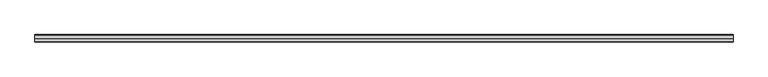
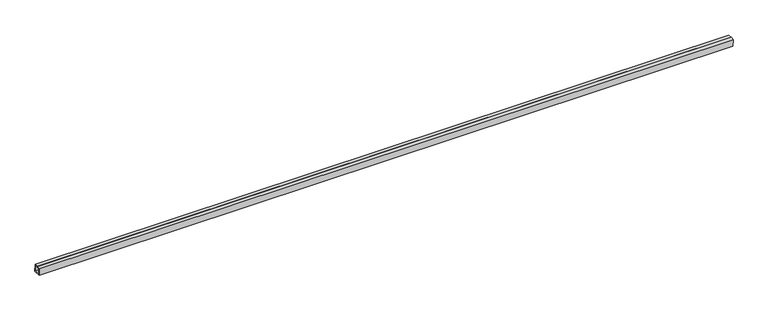
"""IFC4 building model written with IfcOpenShell, lengths in millimetres: proxy geometry, Inner panel:Inner panel:1:Inner panel:1 : Inner panel:Inner panel:300324:2:Inner panel:1:Inner panel:1 : Inner panel:Inner panel:300324:2 : Inner panel:Inner panel:1:Inner panel:1 : Inner panel:Inner panel:300324:300043:42 : Inner panel:Inner panel:1:Inner panel:1 : Inner panel:Inner panel:300324:2:Inner panel:1:Inner panel:1 : Inner panel:Inner panel:300324:2 : Inner panel:Inner panel:1:Inner panel:1 : Inner panel:Inner panel:300324:300043:308120."""

from ifc_helpers import new_model, si_unit, frame, origin, place, context, project, spatial, polyline, outline, extrude, source, transform, mapped, element, save


def generic_models_dc7f755b(model_context):
    return source(origin(), model_context, "Body", "SweptSolid", [
        extrude(outline(polyline([(-577258.3887241, 4022.4942957), (-577240.148301, 4023.2543133), (-577238.5621772, 3985.1873432), (-577276.6291473, 3983.6012194), (-577278.215271, 4021.6681895), (-577259.9748479, 4022.4282072), (-577259.8757151, 4020.0490215), (-577275.7369527, 4019.3881366), (-577274.3490944, 3986.0795378), (-577241.0404956, 3987.4673961), (-577242.4283539, 4020.7759949), (-577258.2895914, 4020.11511), (-577258.3887241, 4022.4942957)])), frame((612749.9867239, 0.0, 0.0), z_axis=(1.0, 0.0, 0.0), x_axis=(0.0, 1.0, 0.0)), (0.0, 0.0, 1.0), 3657.6),
    ])


if __name__ == "__main__":
    model = new_model("IFC4")
    model_context = context("Model", 3, world=origin())
    ifc_project = project(units=[si_unit("LENGTHUNIT", "METRE", prefix="MILLI")], contexts=[model_context])
    site = spatial("IfcSite", under=ifc_project)
    building = spatial("IfcBuilding", under=site)
    placement = place(None, origin())
    generic_models_shape = generic_models_dc7f755b(model_context)
    element("IfcBuildingElementProxy", 1, Name="Inner panel:Inner panel:1:Inner panel:1 : Inner panel:Inner panel:300324:2:Inner panel:1:Inner panel:1 : Inner panel:Inner panel:300324:2 : Inner panel:Inner panel:1:Inner panel:1 : Inner panel:Inner panel:300324:300043:42 : Inner panel:Inner panel:1:Inner panel:1 : Inner panel:Inner panel:300324:2:Inner panel:1:Inner panel:1 : Inner panel:Inner panel:300324:2 : Inner panel:Inner panel:1:Inner panel:1 : Inner panel:Inner panel:300324:300043:308120", ObjectType="Inner panel:Inner panel:1:Inner panel:1 : Inner panel:Inner panel:300324:2:Inner panel:1:Inner panel:1 : Inner panel:Inner panel:300324:2 : Inner panel:Inner panel:1:Inner panel:1 : Inner panel:Inner panel:300324:300043:42 : Inner panel:Inner panel:1:Inner panel:1 : Inner panel:Inner panel:300324:2:Inner panel:1:Inner panel:1 : Inner panel:Inner panel:300324:2 : Inner panel:Inner panel:1:Inner panel:1 : Inner panel:Inner panel:300324:300043:308120", at=placement, inside=building, context=model_context, shape_type="MappedRepresentation", body=[
        mapped(generic_models_shape, transform((0.0, 0.0, 0.0), x_axis=(1.0, 0.0, 0.0), y_axis=(0.0, 1.0, 0.0), z_axis=(0.0, 0.0, 1.0))),
    ])
    save(model, "model.ifc")

# Revit data of these elements
# Type "Inner panel:Inner panel:1:Inner panel:1 : Inner panel:Inner panel:300324:2:Inner panel:1:Inner panel:1 : Inner panel:Inner panel:300324:2 : Inner panel:Inner panel:1:Inner panel:1 : Inner panel:Inner panel:300324:300043:42 : Inner panel:Inner panel:1:Inner panel:1 : Inner panel:Inner panel:300324:2:Inner panel:1:Inner panel:1 : Inner panel:Inner panel:300324:2 : Inner panel:Inner panel:1:Inner panel:1 : Inner panel:Inner panel:300324:300043:308120"
#   NameOverride = "Inner panel:Inner panel:1:Inner panel:1 : Inner panel:Inner panel:300324:2:Inner panel:1:Inner panel:1 : Inner panel:Inner panel:300324:2 : Inner panel:Inner panel:1:Inner panel:1 : Inner panel:Inner panel:300324:300043:308120"
#   ObjectTypeOverride = "Inner panel:1:Inner panel:1 : Inner panel:Inner panel:300324:2 : Inner panel:Inner panel:1:Inner panel:1 : Inner panel:Inner panel:300324:300043"
#   Reference = "Inner panel"
#   Tag = "308120"
# Element 1 (IfcBuildingElementProxy, "Inner panel:Inner panel:1:Inner panel:1 : Inner panel:Inner panel:300324:2:Inner panel:1:Inner panel:1 : Inner panel:Inner panel:300324:2 : Inner panel:Inner panel:1:Inner panel:1 : Inner panel:Inner panel:300324:300043:42 : Inner panel:Inner panel:1:Inner panel:1 : Inner panel:Inner panel:300324:2:Inner panel:1:Inner panel:1 : Inner panel:Inner panel:300324:2 : Inner panel:Inner panel:1:Inner panel:1 : Inner panel:Inner panel:300324:300043:308120")
#   Materials on its faces: "1 1/2\" X 1 1/2\" SPLIT-SEAM SQUARE TUBING (~24\" CANTILEVER FROM C.L. OF GLULAM)"
# Materials
#   "1 1/2\" X 1 1/2\" SPLIT-SEAM SQUARE TUBING (~24\" CANTILEVER FROM C.L. OF GLULAM)": class "Unassigned", colour RGB 202 201 200, transparency 0, Cost = 0
